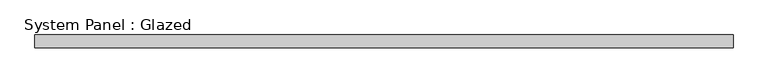
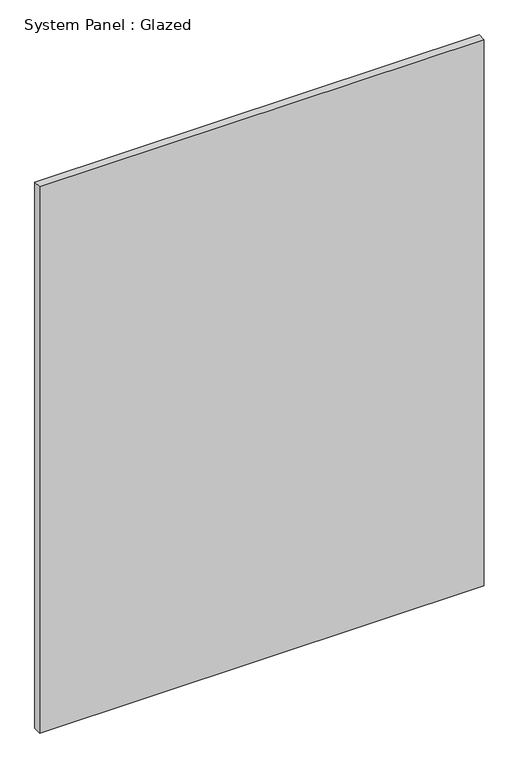
"""IFC4 building model written with IfcOpenShell, lengths in millimetres: plate geometry, System Panel : Glazed."""

from ifc_helpers import new_model, si_unit, origin, origin_with_axes, place, context, project, spatial, polyline, outline, extrude, source, transform, mapped, element, save


def system_panel_glazed_2616a3f9(model_context):
    return source(origin(), model_context, "Body", "SweptSolid", [
        extrude(outline(polyline([(682.4999999, 24.5), (-682.4999999, 24.5), (-682.4999999, 49.5), (682.4999999, 49.5), (682.4999999, 24.5)])), origin_with_axes(), (0.0, 0.0, 1.0), 1772.3836314),
    ])


if __name__ == "__main__":
    model = new_model("IFC4")
    model_context = context("Model", 3, world=origin())
    ifc_project = project(units=[si_unit("LENGTHUNIT", "METRE", prefix="MILLI")], contexts=[model_context])
    site = spatial("IfcSite", under=ifc_project)
    building = spatial("IfcBuilding", under=site)
    placement = place(None, origin())
    system_panel_glazed_shape = system_panel_glazed_2616a3f9(model_context)
    element("IfcPlate", 1, ObjectType="System Panel : Glazed", at=placement, inside=building, context=model_context, shape_type="MappedRepresentation", body=[
        mapped(system_panel_glazed_shape, transform((0.0, 0.0, 0.0), x_axis=(1.0, 0.0, 0.0), y_axis=(0.0, 1.0, 0.0), z_axis=(0.0, 0.0, 1.0))),
    ])
    save(model, "model.ifc")

# Revit data of these elements
# Element 1 (IfcPlate, "System Panel : Glazed")
#   Materials on its faces: "Glass"
# Materials
#   "Glass": class "Glass", colour RGB 218 227 224, transparency 0.85, Description = "Soda Lime Glass", Cost = 0
